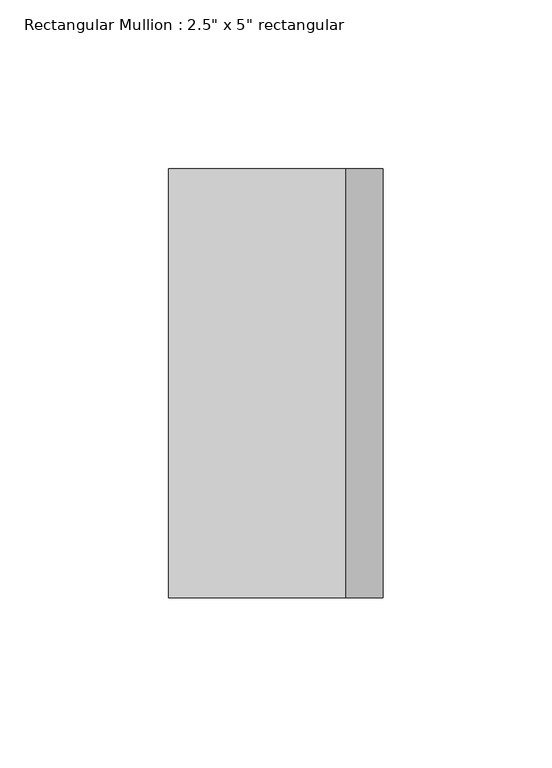
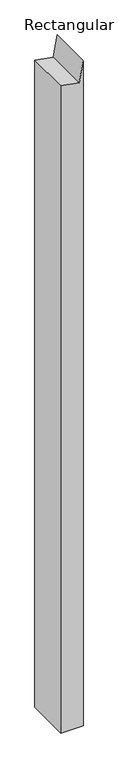
"""IFC4 building model written with IfcOpenShell, lengths in millimetres: member geometry."""

from ifc_helpers import new_model, si_unit, frame, origin, place, context, project, spatial, polyline, outline, extrude, source, transform, mapped, element, save


def member_1b0e919a(model_context):
    return source(origin(), model_context, "Body", "SweptSolid", [
        extrude(outline(polyline([(0.0, 0.0), (-62.5352923, -11.0266593), (-53.2828266, -63.5), (-1997.6226708, -63.5), (-1997.6226708, 0.0), (0.0, 0.0)])), frame((0.0, -63.5, 0.0), z_axis=(0.0, 1.0, 0.0), x_axis=(0.0, 0.0, 1.0)), (0.0, 0.0, 1.0), 127.0),
    ])


if __name__ == "__main__":
    model = new_model("IFC4")
    model_context = context("Model", 3, world=origin())
    ifc_project = project(units=[si_unit("LENGTHUNIT", "METRE", prefix="MILLI")], contexts=[model_context])
    site = spatial("IfcSite", under=ifc_project)
    building = spatial("IfcBuilding", under=site)
    placement = place(None, origin())
    member_shape = member_1b0e919a(model_context)
    element("IfcMember", 1, ObjectType="Rectangular Mullion : 2.5\" x 5\" rectangular", at=placement, inside=building, context=model_context, shape_type="MappedRepresentation", body=[
        mapped(member_shape, transform((0.0, 0.0, 0.0), x_axis=(1.0, 0.0, 0.0), y_axis=(0.0, 1.0, 0.0), z_axis=(0.0, 0.0, 1.0))),
    ])
    save(model, "model.ifc")

# Revit data of these elements
# Type "Rectangular Mullion : 2.5\" x 5\" rectangular"
#   built-in parameter 1007304 = 0.416667 (stored number, unit not read)
#   built-in parameter 1007301 = 0.104167 (stored number, unit not read)
#   built-in parameter 1007300 = 0.104167 (stored number, unit not read)
# Element 1 (IfcMember, "Rectangular Mullion : 2.5\" x 5\" rectangular")
#   Materials on its faces: "Black Mullions"
# Materials
#   "Black Mullions": class "Wood", colour RGB 0 0 0, transparency 0, Cost = 0
